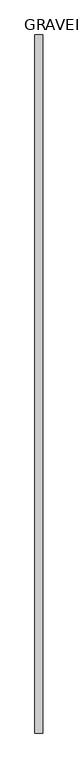
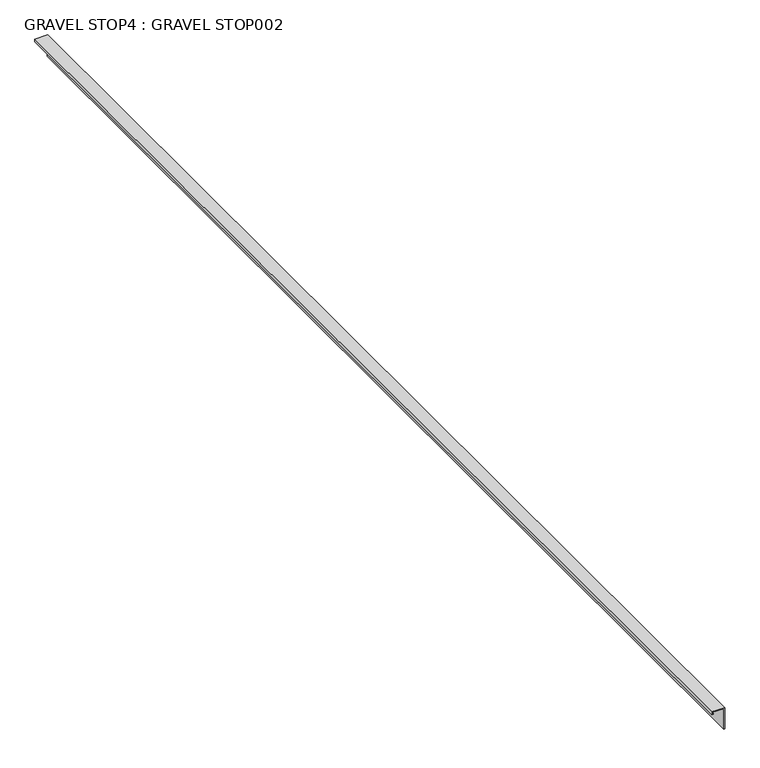
"""IFC4 building model written with IfcOpenShell, lengths in millimetres: proxy geometry, GRAVEL STOP4 : GRAVEL STOP002."""

from ifc_helpers import new_model, si_unit, frame, origin, place, context, project, spatial, polyline, outline, extrude, source, transform, mapped, element, save


def gravel_stop4_gravel_stop002_7d4a8986(model_context):
    return source(origin(), model_context, "Body", "SweptSolid", [
        extrude(outline(polyline([(40234.4061757, -2790.7286469), (40197.5761757, -2790.7286469), (40197.5761757, -2789.4586469), (40235.6761757, -2789.4586469), (40235.6761757, -2811.6836469), (40230.9263757, -2811.6836469), (40230.9263757, -2808.6811906), (40232.1963757, -2808.6811906), (40232.1963757, -2810.4136469), (40234.4061757, -2810.4136469), (40234.4061757, -2790.7286469)])), frame((0.0, 1000.0000001, 0.0), z_axis=(0.0, 1.0, 0.0), x_axis=(0.0, 0.0, 1.0)), (0.0, 0.0, 1.0), 2000.25),
    ])


if __name__ == "__main__":
    model = new_model("IFC4")
    model_context = context("Model", 3, world=origin())
    ifc_project = project(units=[si_unit("LENGTHUNIT", "METRE", prefix="MILLI")], contexts=[model_context])
    site = spatial("IfcSite", under=ifc_project)
    building = spatial("IfcBuilding", under=site)
    placement = place(None, origin())
    gravel_stop4_gravel_stop002_shape = gravel_stop4_gravel_stop002_7d4a8986(model_context)
    element("IfcBuildingElementProxy", 1, Name="GRAVEL STOP4 : GRAVEL STOP002", ObjectType="GRAVEL STOP4 : GRAVEL STOP002", at=placement, inside=building, context=model_context, shape_type="MappedRepresentation", body=[
        mapped(gravel_stop4_gravel_stop002_shape, transform((0.0, 0.0, 0.0), x_axis=(1.0, 0.0, 0.0), y_axis=(0.0, 1.0, 0.0), z_axis=(0.0, 0.0, 1.0))),
    ])
    save(model, "model.ifc")

# Revit data of these elements
# Type "GRAVEL STOP4 : GRAVEL STOP002"
#   NameOverride = "GRAVEL STOP002"
# Element 1 (IfcBuildingElementProxy, "GRAVEL STOP4 : GRAVEL STOP002")
#   Materials on its faces: "COPPER STUCCO J BEAD"
# Materials
#   "COPPER STUCCO J BEAD": class "Unassigned", colour RGB 251 232 155, transparency 0, Cost = 0
